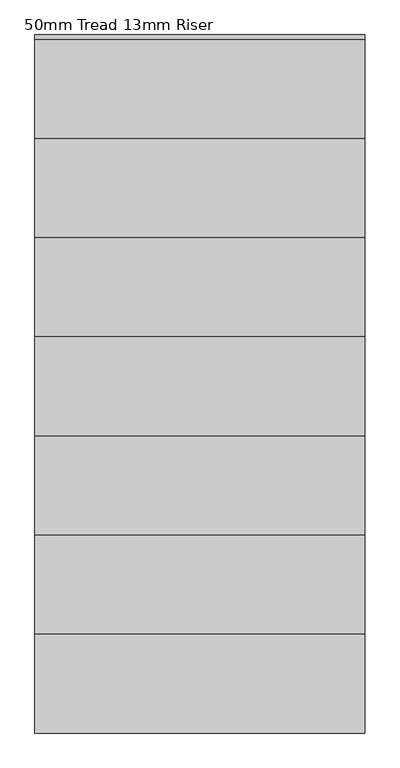
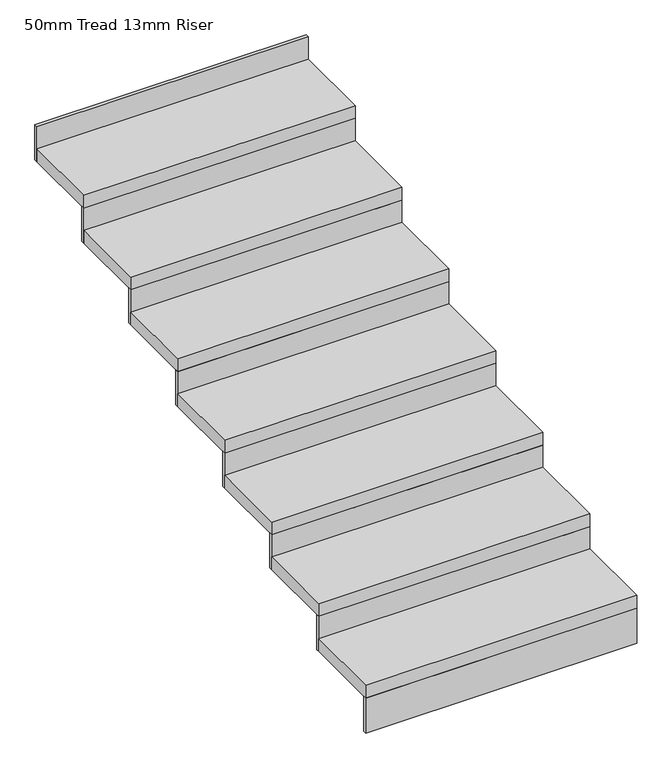
"""IFC4 building model written with IfcOpenShell, lengths in millimetres: stair flight geometry, 50mm Tread 13mm Riser."""

from ifc_helpers import new_model, si_unit, frame, origin, place, context, project, spatial, polyline, outline, extrude, source, transform, mapped, element, save


def stair_flight_50mm_tread_13mm_riser_a7928dec(model_context):
    return source(origin(), model_context, "Body", "SweptSolid", [
        extrude(outline(polyline([(22529.836337, -2888.024372), (22529.836337, -2900.524372), (21529.836337, -2900.524372), (21529.836337, -2888.024372), (22529.836337, -2888.024372)])), frame((0.0, 0.0, 1859.0909091), z_axis=(0.0, 0.0, 1.0), x_axis=(1.0, 0.0, 0.0)), (0.0, 0.0, 1.0), 136.3636364),
        extrude(outline(polyline([(21529.836337, -2600.524372), (22529.836337, -2600.524372), (22529.836337, -2900.524372), (21529.836337, -2900.524372), (21529.836337, -2600.524372)])), frame((0.0, 0.0, 1995.4545455), z_axis=(0.0, 0.0, 1.0), x_axis=(1.0, 0.0, 0.0)), (0.0, 0.0, 1.0), 50.0),
        extrude(outline(polyline([(22529.836337, -2588.024372), (22529.836337, -2600.524372), (21529.836337, -2600.524372), (21529.836337, -2588.024372), (22529.836337, -2588.024372)])), frame((0.0, 0.0, 1995.4545455), z_axis=(0.0, 0.0, 1.0), x_axis=(1.0, 0.0, 0.0)), (0.0, 0.0, 1.0), 136.3636364),
        extrude(outline(polyline([(21529.836337, -2300.524372), (22529.836337, -2300.524372), (22529.836337, -2600.524372), (21529.836337, -2600.524372), (21529.836337, -2300.524372)])), frame((0.0, 0.0, 2131.8181818), z_axis=(0.0, 0.0, 1.0), x_axis=(1.0, 0.0, 0.0)), (0.0, 0.0, 1.0), 50.0),
        extrude(outline(polyline([(22529.836337, -2288.024372), (22529.836337, -2300.524372), (21529.836337, -2300.524372), (21529.836337, -2288.024372), (22529.836337, -2288.024372)])), frame((0.0, 0.0, 2131.8181818), z_axis=(0.0, 0.0, 1.0), x_axis=(1.0, 0.0, 0.0)), (0.0, 0.0, 1.0), 136.3636364),
        extrude(outline(polyline([(21529.836337, -2000.524372), (22529.836337, -2000.524372), (22529.836337, -2300.524372), (21529.836337, -2300.524372), (21529.836337, -2000.524372)])), frame((0.0, 0.0, 2268.1818182), z_axis=(0.0, 0.0, 1.0), x_axis=(1.0, 0.0, 0.0)), (0.0, 0.0, 1.0), 50.0),
        extrude(outline(polyline([(22529.836337, -1988.024372), (22529.836337, -2000.524372), (21529.836337, -2000.524372), (21529.836337, -1988.024372), (22529.836337, -1988.024372)])), frame((0.0, 0.0, 2268.1818182), z_axis=(0.0, 0.0, 1.0), x_axis=(1.0, 0.0, 0.0)), (0.0, 0.0, 1.0), 136.3636364),
        extrude(outline(polyline([(21529.836337, -1700.524372), (22529.836337, -1700.524372), (22529.836337, -2000.524372), (21529.836337, -2000.524372), (21529.836337, -1700.524372)])), frame((0.0, 0.0, 2404.5454545), z_axis=(0.0, 0.0, 1.0), x_axis=(1.0, 0.0, 0.0)), (0.0, 0.0, 1.0), 50.0),
        extrude(outline(polyline([(22529.836337, -1688.024372), (22529.836337, -1700.524372), (21529.836337, -1700.524372), (21529.836337, -1688.024372), (22529.836337, -1688.024372)])), frame((0.0, 0.0, 2404.5454545), z_axis=(0.0, 0.0, 1.0), x_axis=(1.0, 0.0, 0.0)), (0.0, 0.0, 1.0), 136.3636364),
        extrude(outline(polyline([(21529.836337, -1400.524372), (22529.836337, -1400.524372), (22529.836337, -1700.524372), (21529.836337, -1700.524372), (21529.836337, -1400.524372)])), frame((0.0, 0.0, 2540.9090909), z_axis=(0.0, 0.0, 1.0), x_axis=(1.0, 0.0, 0.0)), (0.0, 0.0, 1.0), 50.0),
        extrude(outline(polyline([(22529.836337, -1388.024372), (22529.836337, -1400.524372), (21529.836337, -1400.524372), (21529.836337, -1388.024372), (22529.836337, -1388.024372)])), frame((0.0, 0.0, 2540.9090909), z_axis=(0.0, 0.0, 1.0), x_axis=(1.0, 0.0, 0.0)), (0.0, 0.0, 1.0), 136.3636364),
        extrude(outline(polyline([(21529.836337, -1100.524372), (22529.836337, -1100.524372), (22529.836337, -1400.524372), (21529.836337, -1400.524372), (21529.836337, -1100.524372)])), frame((0.0, 0.0, 2677.2727273), z_axis=(0.0, 0.0, 1.0), x_axis=(1.0, 0.0, 0.0)), (0.0, 0.0, 1.0), 50.0),
        extrude(outline(polyline([(22529.836337, -1088.024372), (22529.836337, -1100.524372), (21529.836337, -1100.524372), (21529.836337, -1088.024372), (22529.836337, -1088.024372)])), frame((0.0, 0.0, 2677.2727273), z_axis=(0.0, 0.0, 1.0), x_axis=(1.0, 0.0, 0.0)), (0.0, 0.0, 1.0), 136.3636364),
        extrude(outline(polyline([(21529.836337, -800.524372), (22529.836337, -800.524372), (22529.836337, -1100.524372), (21529.836337, -1100.524372), (21529.836337, -800.524372)])), frame((0.0, 0.0, 2813.6363636), z_axis=(0.0, 0.0, 1.0), x_axis=(1.0, 0.0, 0.0)), (0.0, 0.0, 1.0), 50.0),
        extrude(outline(polyline([(22529.836337, -788.024372), (22529.836337, -800.524372), (21529.836337, -800.524372), (21529.836337, -788.024372), (22529.836337, -788.024372)])), frame((0.0, 0.0, 2813.6363636), z_axis=(0.0, 0.0, 1.0), x_axis=(1.0, 0.0, 0.0)), (0.0, 0.0, 1.0), 136.3636364),
    ])


if __name__ == "__main__":
    model = new_model("IFC4")
    model_context = context("Model", 3, world=origin())
    ifc_project = project(units=[si_unit("LENGTHUNIT", "METRE", prefix="MILLI")], contexts=[model_context])
    site = spatial("IfcSite", under=ifc_project)
    building = spatial("IfcBuilding", under=site)
    placement = place(None, origin())
    stair_flight_50mm_tread_13mm_riser_shape = stair_flight_50mm_tread_13mm_riser_a7928dec(model_context)
    element("IfcStairFlight", 1, ObjectType="50mm Tread 13mm Riser", at=placement, inside=building, context=model_context, shape_type="MappedRepresentation", body=[
        mapped(stair_flight_50mm_tread_13mm_riser_shape, transform((0.0, 0.0, 0.0), x_axis=(1.0, 0.0, 0.0), y_axis=(0.0, 1.0, 0.0), z_axis=(0.0, 0.0, 1.0))),
    ])
    save(model, "model.ifc")
